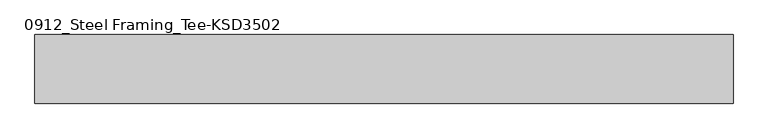
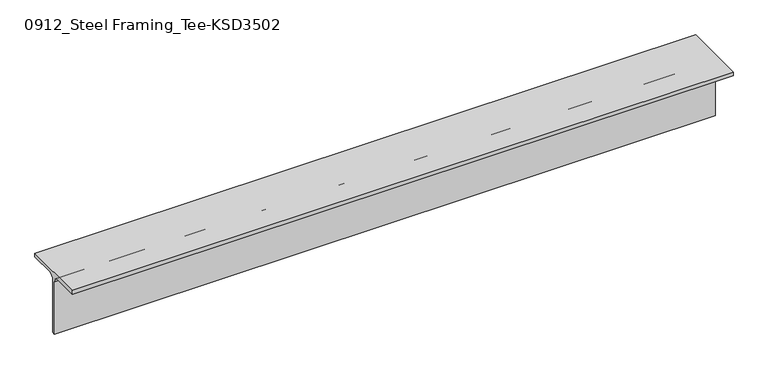
"""IFC4 building model written with IfcOpenShell, lengths in millimetres: member geometry, 0912_Steel Framing_Tee-KSD3502 : H_SB_ASB_CT-150x150x6.5x9."""

import ifcopenshell
import ifcopenshell.guid

model = None  # the IFC model being written
_history = None  # IfcOwnerHistory: only IFC2X3 demands one
_inside = {}  # id of a spatial element -> (the spatial element, [elements in it])
_under = {}  # id of a project, library or spatial element -> (it, [spatial elements below it])
_declared = {}  # id of a project -> (the project, [libraries it declares])
_typed = {}  # id of a type object -> (the type object, [elements of that type])
_made_of = {}  # id of a material, layer set ... -> (it, [elements and type objects made of it])


def new_model(schema):
    """Start an empty IFC model of exactly this schema.

    Asked for "IFC4X3", IfcOpenShell would pick the latest addendum, in which some entities
    have other attributes; the version numbers below select the first issue.
    IFC2X3 requires an IfcOwnerHistory on every rooted entity: one is made here for all.
    """
    global model, _history
    if schema == "IFC4X3":
        model = ifcopenshell.file(schema_version=(4, 3, 0, 0))
    else:
        model = ifcopenshell.file(schema=schema)
    _inside.clear()
    _under.clear()
    _declared.clear()
    _typed.clear()
    _made_of.clear()
    _history = None
    if model.schema == "IFC2X3":
        org = make("IfcOrganization", Name="unknown")
        user = make(
            "IfcPersonAndOrganization",
            ThePerson=make("IfcPerson", FamilyName="unknown"),
            TheOrganization=org,
        )
        app = make(
            "IfcApplication",
            ApplicationDeveloper=org,
            Version="unknown",
            ApplicationFullName="unknown",
            ApplicationIdentifier="unknown",
        )
        _history = make(
            "IfcOwnerHistory",
            OwningUser=user,
            OwningApplication=app,
            ChangeAction="ADDED",
            CreationDate=0,
        )
    return model


def make(cls, **values):
    """One entity of the class cls with the attributes given. An attribute that is None is left unset."""
    return model.create_entity(
        cls, **{name: value for name, value in values.items() if value is not None}
    )


def rooted(cls, **values):
    """An entity with a GlobalId (a new one), such as an element, a storey or a relation."""
    return make(cls, GlobalId=ifcopenshell.guid.new(), OwnerHistory=_history, **values)


def si_unit(unit_type, name, prefix=None):
    """IfcSIUnit, for example si_unit("LENGTHUNIT", "METRE", prefix="MILLI")."""
    return make("IfcSIUnit", UnitType=unit_type, Prefix=prefix, Name=name)


def assignment(units):
    """IfcUnitAssignment: the units of a project."""
    return None if units is None else make("IfcUnitAssignment", Units=units)


def point(xyz):
    """IfcCartesianPoint."""
    return None if xyz is None else make("IfcCartesianPoint", Coordinates=xyz)


def direction(xyz):
    """IfcDirection."""
    return None if xyz is None else make("IfcDirection", DirectionRatios=xyz)


def frame(location, z_axis=None, x_axis=None):
    """IfcAxis2Placement3D, a coordinate frame: its origin and axes. An axis left out is left unset."""
    return make(
        "IfcAxis2Placement3D",
        Location=point(location),
        Axis=direction(z_axis),
        RefDirection=direction(x_axis),
    )


def frame_2d(location, x_axis=None):
    """IfcAxis2Placement2D, a coordinate frame in the plane: its origin and x axis."""
    return make(
        "IfcAxis2Placement2D", Location=point(location), RefDirection=direction(x_axis)
    )


def origin():
    """The frame at (0, 0, 0) with its axes left unset."""
    return frame((0.0, 0.0, 0.0))


def place(relative_to, where):
    """IfcLocalPlacement: puts the frame where relative to a parent placement (None: the world)."""
    return make(
        "IfcLocalPlacement", PlacementRelTo=relative_to, RelativePlacement=where
    )


def context(
    kind, dimensions, precision=None, world=None, true_north=None, identifier=None
):
    """IfcGeometricRepresentationContext, for example the 3D "Model" context."""
    return make(
        "IfcGeometricRepresentationContext",
        ContextIdentifier=identifier,
        ContextType=kind,
        CoordinateSpaceDimension=dimensions,
        Precision=precision,
        WorldCoordinateSystem=world,
        TrueNorth=true_north,
    )


def project(units=None, contexts=None):
    """IfcProject with its units and contexts."""
    return rooted(
        "IfcProject",
        Name="project",
        RepresentationContexts=contexts,
        UnitsInContext=assignment(units),
    )


def spatial(cls, under=None, at=None, **own):
    """A site, building, storey or space (cls), placed at a placement, below another one or the project."""
    s = rooted(cls, ObjectPlacement=at, **own)
    if under is not None:
        _under.setdefault(under.id(), (under, []))[1].append(s)
    return s


def polyline(points):
    """IfcPolyline through the points."""
    return make("IfcPolyline", Points=[point(p) for p in points])


def circle_curve(where, radius):
    """IfcCircle in the frame where."""
    return make("IfcCircle", Position=where, Radius=radius)


def trimmed(basis, trim1, trim2, sense, master):
    """IfcTrimmedCurve: the piece of a basis curve between two trims."""
    return make(
        "IfcTrimmedCurve",
        BasisCurve=basis,
        Trim1=trim1,
        Trim2=trim2,
        SenseAgreement=sense,
        MasterRepresentation=master,
    )


def segment(curve, same_sense, transition):
    """IfcCompositeCurveSegment."""
    return make(
        "IfcCompositeCurveSegment",
        Transition=transition,
        SameSense=same_sense,
        ParentCurve=curve,
    )


def composite_curve(segments, self_intersect=None):
    """IfcCompositeCurve: segments joined end to end."""
    return make("IfcCompositeCurve", Segments=segments, SelfIntersect=self_intersect)


def outline(outer, holes=None, kind="AREA"):
    """IfcArbitraryClosedProfileDef: a profile drawn as a closed curve; with holes, ...WithVoids."""
    if holes is None:
        return make("IfcArbitraryClosedProfileDef", ProfileType=kind, OuterCurve=outer)
    return make(
        "IfcArbitraryProfileDefWithVoids",
        ProfileType=kind,
        OuterCurve=outer,
        InnerCurves=holes,
    )


def extrude(swept, where, along, depth):
    """IfcExtrudedAreaSolid: the profile swept, set in the frame where, extruded along a direction by depth."""
    return make(
        "IfcExtrudedAreaSolid",
        SweptArea=swept,
        Position=where,
        ExtrudedDirection=direction(along),
        Depth=depth,
    )


def shape(context_of_items, identifier, shape_type, items):
    """IfcShapeRepresentation: the items that make up one representation, for example the "Body"."""
    return make(
        "IfcShapeRepresentation",
        ContextOfItems=context_of_items,
        RepresentationIdentifier=identifier,
        RepresentationType=shape_type,
        Items=items,
    )


def source(mapping_origin, context_of_items, identifier, shape_type, items):
    """IfcRepresentationMap: a shape defined once, which mapped items show again and again."""
    return make(
        "IfcRepresentationMap",
        MappingOrigin=mapping_origin,
        MappedRepresentation=shape(context_of_items, identifier, shape_type, items),
    )


def transform(
    local_origin,
    x_axis=None,
    y_axis=None,
    z_axis=None,
    scale=None,
    scale2=None,
    scale3=None,
    uniform=True,
):
    """IfcCartesianTransformationOperator3D, or its non-uniform kind. x_axis, y_axis, z_axis: its Axis1, 2, 3."""
    if uniform:
        return make(
            "IfcCartesianTransformationOperator3D",
            Axis1=direction(x_axis),
            Axis2=direction(y_axis),
            LocalOrigin=point(local_origin),
            Scale=scale,
            Axis3=direction(z_axis),
        )
    return make(
        "IfcCartesianTransformationOperator3DnonUniform",
        Axis1=direction(x_axis),
        Axis2=direction(y_axis),
        LocalOrigin=point(local_origin),
        Scale=scale,
        Axis3=direction(z_axis),
        Scale2=scale2,
        Scale3=scale3,
    )


def mapped(mapping_source, mapping_target):
    """IfcMappedItem: shows the shape of a source again, moved by a transform."""
    return make(
        "IfcMappedItem", MappingSource=mapping_source, MappingTarget=mapping_target
    )


def made_of(thing, what):
    """Note that an element or type object is made of a material, layer set ...; save() writes the relation."""
    if what is not None:
        _made_of.setdefault(what.id(), (what, []))[1].append(thing)
    return thing


def element(
    cls,
    number,
    at=None,
    inside=None,
    cuts=None,
    type_object=None,
    material=None,
    context=None,
    identifier="Body",
    shape_type=None,
    held_by="IfcProductDefinitionShape",
    body=None,
    shapes=None,
    **own,
):
    """One element of the class cls, such as IfcWall. Its Tag is "e" and its number.

    at: its placement. inside: the storey or other place that contains it. cuts: it is an
    opening in that element (IfcRelVoidsElement). A single representation is given by context,
    identifier, shape_type and body (its items); several are given by shapes. held_by: the class
    of the entity that holds the representations. save() writes the other relations.
    """
    e = rooted(cls, Tag="e%d" % number, ObjectPlacement=at, **own)
    if body is not None:
        shapes = [shape(context, identifier, shape_type, body)]
    if shapes is not None:
        e.Representation = make(held_by, Representations=shapes)
    if inside is not None:
        _inside.setdefault(inside.id(), (inside, []))[1].append(e)
    if cuts is not None:
        rooted(
            "IfcRelVoidsElement", RelatingBuildingElement=cuts, RelatedOpeningElement=e
        )
    if type_object is not None:
        _typed.setdefault(type_object.id(), (type_object, []))[1].append(e)
    return made_of(e, material)


def aggregate(whole, parts):
    """IfcRelAggregates: a whole, such as a stair, and the parts it consists of."""
    return rooted("IfcRelAggregates", RelatingObject=whole, RelatedObjects=parts)


def save(model, path):
    """Write the relations noted so far, then the file.

    IfcRelAggregates (storeys below a building ...), IfcRelContainedInSpatialStructure (elements
    in a storey), IfcRelDefinesByType, IfcRelAssociatesMaterial and IfcRelDeclares: one each for
    every whole, place, type object, material and project.
    """
    for whole, parts in _under.values():
        aggregate(whole, parts)
    for where, things in _inside.values():
        rooted(
            "IfcRelContainedInSpatialStructure",
            RelatedElements=things,
            RelatingStructure=where,
        )
    for kind, things in _typed.values():
        rooted("IfcRelDefinesByType", RelatedObjects=things, RelatingType=kind)
    for what, things in _made_of.values():
        rooted("IfcRelAssociatesMaterial", RelatedObjects=things, RelatingMaterial=what)
    for by, libraries in _declared.values():
        rooted("IfcRelDeclares", RelatingContext=by, RelatedDefinitions=libraries)
    model.write(path)


def member_0912_steel_framing_tee_ksd3502_3a543eb5(model_context):
    return source(origin(), model_context, "Body", "SweptSolid", [
        extrude(outline(composite_curve([segment(polyline([(-75.0, 75.0), (75.0, 75.0), (75.0, 66.0), (16.25, 66.0)]), True, "CONTINUOUS"), segment(trimmed(circle_curve(frame_2d((16.25, 53.0)), 13.0), [point((16.25, 66.0))], [point((3.25, 53.0))], True, "CARTESIAN"), True, "CONTINUOUS"), segment(polyline([(3.25, 53.0), (3.25, -75.0), (-3.25, -75.0), (-3.25, 53.0)]), True, "CONTINUOUS"), segment(trimmed(circle_curve(frame_2d((-16.25, 53.0)), 13.0), [point((-3.25, 53.0))], [point((-16.25, 66.0))], True, "CARTESIAN"), True, "CONTINUOUS"), segment(polyline([(-16.25, 66.0), (-75.0, 66.0), (-75.0, 75.0)]), True, "CONTINUOUS")], self_intersect=False)), frame((-719.0, 0.0, 0.0), z_axis=(1.0, 0.0, 0.0), x_axis=(0.0, 1.0, 0.0)), (0.0, 0.0, 1.0), 1526.1),
    ])


if __name__ == "__main__":
    model = new_model("IFC4")
    model_context = context("Model", 3, world=origin())
    ifc_project = project(units=[si_unit("LENGTHUNIT", "METRE", prefix="MILLI")], contexts=[model_context])
    site = spatial("IfcSite", under=ifc_project)
    building = spatial("IfcBuilding", under=site)
    placement = place(None, origin())
    member_0912_steel_framing_tee_ksd3502_shape = member_0912_steel_framing_tee_ksd3502_3a543eb5(model_context)
    element("IfcMember", 1, ObjectType="0912_Steel Framing_Tee-KSD3502 : H_SB_ASB_CT-150x150x6.5x9", at=placement, inside=building, context=model_context, shape_type="MappedRepresentation", body=[
        mapped(member_0912_steel_framing_tee_ksd3502_shape, transform((0.0, 0.0, 0.0), x_axis=(1.0, 0.0, 0.0), y_axis=(0.0, 1.0, 0.0), z_axis=(0.0, 0.0, 1.0))),
    ])
    save(model, "model.ifc")

# Revit data of these elements
# Type "0912_Steel Framing_Tee-KSD3502 : H_SB_ASB_CT-150x150x6.5x9"
#   H_WM Code_1 = "S01AA003-00001 | Main Steel Structure Fabrication Work | Shelter/Building | Light Steel - Standard (30KG/M>Weight) | Material: (   )"
#   H_WM Code_2 = "S03AA029-00001 | Main Steel Structure Erection Work | Shelter/Building | Light Steel (30KG/M>Weight) | Material: (   )"
#   H_WM Code_3 = "S01AA010-00001 | Main Steel Structure Fabrication Work | Shelter/Building | Steel Painting/Coating | for Non-Fireproofed Steel Surface, Surface Preparation, Primer, Second & Final Coat | Material: (   )"
#   H_Q'ty Cal Type Tag = "SB-Q2"
#   Width = 15.0 cm
#   Web Thickness = 0.65 cm
#   Web Fillet = 1.3 cm
#   Section Area = 23.39 cm²
#   Perimeter = 0.60 m²/m
#   Nominal Weight = 18.40 kgf/m
#   Height = 15.0 cm
#   Flange Thickness = 0.9 cm
#   Centroid Vertical = 7.5 cm
#   Centroid Horizontal = 7.5 cm
#   Length [instance default] = 1.5000 m
#   Structural Material [instance default] = Steel, 45-345
#   Warping Constant = (empty or 0)
#   Torsional Moment of Inertia = 0
#   Section Name Key = ""
#   Plastic Modulus weak axis = 0
#   Plastic Modulus strong axis = 0
#   Moment of Inertia weak axis = 0
#   Moment of Inertia strong axis = 0
#   Elastic Modulus weak axis = 0
#   Elastic Modulus strong axis = 0
#   Bolt Spacing = 0
#   Assembly Code = ""
# Element 1 (IfcMember, "0912_Steel Framing_Tee-KSD3502 : H_SB_ASB_CT-150x150x6.5x9")
#   Structural Material = none
# Materials
#   "Steel, 45-345": class "Metal", colour RGB 189 187 185, transparency 0, Description = "Steel 345 MPa", Cost = 0
